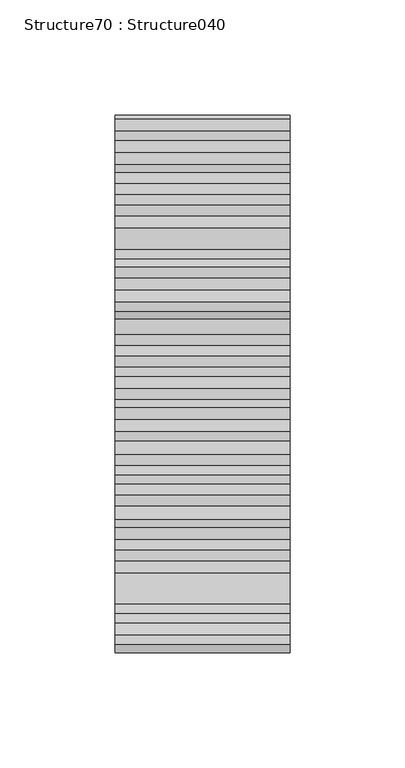
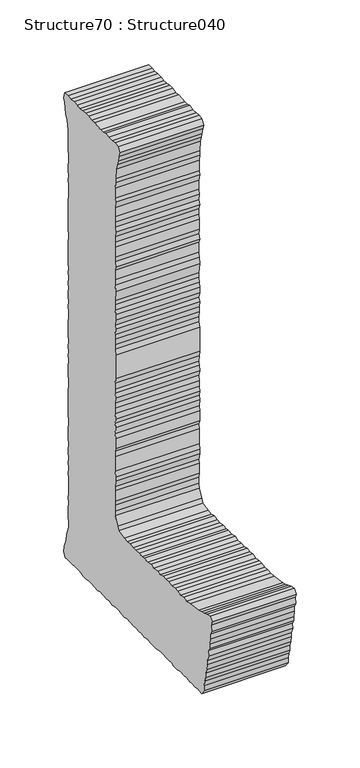
"""IFC4 building model written with IfcOpenShell, lengths in millimetres: proxy geometry, Structure70 : Structure040."""

import ifcopenshell
import ifcopenshell.guid

model = None  # the IFC model being written
_history = None  # IfcOwnerHistory: only IFC2X3 demands one
_inside = {}  # id of a spatial element -> (the spatial element, [elements in it])
_under = {}  # id of a project, library or spatial element -> (it, [spatial elements below it])
_declared = {}  # id of a project -> (the project, [libraries it declares])
_typed = {}  # id of a type object -> (the type object, [elements of that type])
_made_of = {}  # id of a material, layer set ... -> (it, [elements and type objects made of it])


def new_model(schema):
    """Start an empty IFC model of exactly this schema.

    Asked for "IFC4X3", IfcOpenShell would pick the latest addendum, in which some entities
    have other attributes; the version numbers below select the first issue.
    IFC2X3 requires an IfcOwnerHistory on every rooted entity: one is made here for all.
    """
    global model, _history
    if schema == "IFC4X3":
        model = ifcopenshell.file(schema_version=(4, 3, 0, 0))
    else:
        model = ifcopenshell.file(schema=schema)
    _inside.clear()
    _under.clear()
    _declared.clear()
    _typed.clear()
    _made_of.clear()
    _history = None
    if model.schema == "IFC2X3":
        org = make("IfcOrganization", Name="unknown")
        user = make(
            "IfcPersonAndOrganization",
            ThePerson=make("IfcPerson", FamilyName="unknown"),
            TheOrganization=org,
        )
        app = make(
            "IfcApplication",
            ApplicationDeveloper=org,
            Version="unknown",
            ApplicationFullName="unknown",
            ApplicationIdentifier="unknown",
        )
        _history = make(
            "IfcOwnerHistory",
            OwningUser=user,
            OwningApplication=app,
            ChangeAction="ADDED",
            CreationDate=0,
        )
    return model


def make(cls, **values):
    """One entity of the class cls with the attributes given. An attribute that is None is left unset."""
    return model.create_entity(
        cls, **{name: value for name, value in values.items() if value is not None}
    )


def rooted(cls, **values):
    """An entity with a GlobalId (a new one), such as an element, a storey or a relation."""
    return make(cls, GlobalId=ifcopenshell.guid.new(), OwnerHistory=_history, **values)


def si_unit(unit_type, name, prefix=None):
    """IfcSIUnit, for example si_unit("LENGTHUNIT", "METRE", prefix="MILLI")."""
    return make("IfcSIUnit", UnitType=unit_type, Prefix=prefix, Name=name)


def assignment(units):
    """IfcUnitAssignment: the units of a project."""
    return None if units is None else make("IfcUnitAssignment", Units=units)


def point(xyz):
    """IfcCartesianPoint."""
    return None if xyz is None else make("IfcCartesianPoint", Coordinates=xyz)


def direction(xyz):
    """IfcDirection."""
    return None if xyz is None else make("IfcDirection", DirectionRatios=xyz)


def frame(location, z_axis=None, x_axis=None):
    """IfcAxis2Placement3D, a coordinate frame: its origin and axes. An axis left out is left unset."""
    return make(
        "IfcAxis2Placement3D",
        Location=point(location),
        Axis=direction(z_axis),
        RefDirection=direction(x_axis),
    )


def origin():
    """The frame at (0, 0, 0) with its axes left unset."""
    return frame((0.0, 0.0, 0.0))


def place(relative_to, where):
    """IfcLocalPlacement: puts the frame where relative to a parent placement (None: the world)."""
    return make(
        "IfcLocalPlacement", PlacementRelTo=relative_to, RelativePlacement=where
    )


def context(
    kind, dimensions, precision=None, world=None, true_north=None, identifier=None
):
    """IfcGeometricRepresentationContext, for example the 3D "Model" context."""
    return make(
        "IfcGeometricRepresentationContext",
        ContextIdentifier=identifier,
        ContextType=kind,
        CoordinateSpaceDimension=dimensions,
        Precision=precision,
        WorldCoordinateSystem=world,
        TrueNorth=true_north,
    )


def project(units=None, contexts=None):
    """IfcProject with its units and contexts."""
    return rooted(
        "IfcProject",
        Name="project",
        RepresentationContexts=contexts,
        UnitsInContext=assignment(units),
    )


def spatial(cls, under=None, at=None, **own):
    """A site, building, storey or space (cls), placed at a placement, below another one or the project."""
    s = rooted(cls, ObjectPlacement=at, **own)
    if under is not None:
        _under.setdefault(under.id(), (under, []))[1].append(s)
    return s


def polyline(points):
    """IfcPolyline through the points."""
    return make("IfcPolyline", Points=[point(p) for p in points])


def outline(outer, holes=None, kind="AREA"):
    """IfcArbitraryClosedProfileDef: a profile drawn as a closed curve; with holes, ...WithVoids."""
    if holes is None:
        return make("IfcArbitraryClosedProfileDef", ProfileType=kind, OuterCurve=outer)
    return make(
        "IfcArbitraryProfileDefWithVoids",
        ProfileType=kind,
        OuterCurve=outer,
        InnerCurves=holes,
    )


def extrude(swept, where, along, depth):
    """IfcExtrudedAreaSolid: the profile swept, set in the frame where, extruded along a direction by depth."""
    return make(
        "IfcExtrudedAreaSolid",
        SweptArea=swept,
        Position=where,
        ExtrudedDirection=direction(along),
        Depth=depth,
    )


def shape(context_of_items, identifier, shape_type, items):
    """IfcShapeRepresentation: the items that make up one representation, for example the "Body"."""
    return make(
        "IfcShapeRepresentation",
        ContextOfItems=context_of_items,
        RepresentationIdentifier=identifier,
        RepresentationType=shape_type,
        Items=items,
    )


def source(mapping_origin, context_of_items, identifier, shape_type, items):
    """IfcRepresentationMap: a shape defined once, which mapped items show again and again."""
    return make(
        "IfcRepresentationMap",
        MappingOrigin=mapping_origin,
        MappedRepresentation=shape(context_of_items, identifier, shape_type, items),
    )


def transform(
    local_origin,
    x_axis=None,
    y_axis=None,
    z_axis=None,
    scale=None,
    scale2=None,
    scale3=None,
    uniform=True,
):
    """IfcCartesianTransformationOperator3D, or its non-uniform kind. x_axis, y_axis, z_axis: its Axis1, 2, 3."""
    if uniform:
        return make(
            "IfcCartesianTransformationOperator3D",
            Axis1=direction(x_axis),
            Axis2=direction(y_axis),
            LocalOrigin=point(local_origin),
            Scale=scale,
            Axis3=direction(z_axis),
        )
    return make(
        "IfcCartesianTransformationOperator3DnonUniform",
        Axis1=direction(x_axis),
        Axis2=direction(y_axis),
        LocalOrigin=point(local_origin),
        Scale=scale,
        Axis3=direction(z_axis),
        Scale2=scale2,
        Scale3=scale3,
    )


def mapped(mapping_source, mapping_target):
    """IfcMappedItem: shows the shape of a source again, moved by a transform."""
    return make(
        "IfcMappedItem", MappingSource=mapping_source, MappingTarget=mapping_target
    )


def made_of(thing, what):
    """Note that an element or type object is made of a material, layer set ...; save() writes the relation."""
    if what is not None:
        _made_of.setdefault(what.id(), (what, []))[1].append(thing)
    return thing


def element(
    cls,
    number,
    at=None,
    inside=None,
    cuts=None,
    type_object=None,
    material=None,
    context=None,
    identifier="Body",
    shape_type=None,
    held_by="IfcProductDefinitionShape",
    body=None,
    shapes=None,
    **own,
):
    """One element of the class cls, such as IfcWall. Its Tag is "e" and its number.

    at: its placement. inside: the storey or other place that contains it. cuts: it is an
    opening in that element (IfcRelVoidsElement). A single representation is given by context,
    identifier, shape_type and body (its items); several are given by shapes. held_by: the class
    of the entity that holds the representations. save() writes the other relations.
    """
    e = rooted(cls, Tag="e%d" % number, ObjectPlacement=at, **own)
    if body is not None:
        shapes = [shape(context, identifier, shape_type, body)]
    if shapes is not None:
        e.Representation = make(held_by, Representations=shapes)
    if inside is not None:
        _inside.setdefault(inside.id(), (inside, []))[1].append(e)
    if cuts is not None:
        rooted(
            "IfcRelVoidsElement", RelatingBuildingElement=cuts, RelatedOpeningElement=e
        )
    if type_object is not None:
        _typed.setdefault(type_object.id(), (type_object, []))[1].append(e)
    return made_of(e, material)


def aggregate(whole, parts):
    """IfcRelAggregates: a whole, such as a stair, and the parts it consists of."""
    return rooted("IfcRelAggregates", RelatingObject=whole, RelatedObjects=parts)


def save(model, path):
    """Write the relations noted so far, then the file.

    IfcRelAggregates (storeys below a building ...), IfcRelContainedInSpatialStructure (elements
    in a storey), IfcRelDefinesByType, IfcRelAssociatesMaterial and IfcRelDeclares: one each for
    every whole, place, type object, material and project.
    """
    for whole, parts in _under.values():
        aggregate(whole, parts)
    for where, things in _inside.values():
        rooted(
            "IfcRelContainedInSpatialStructure",
            RelatedElements=things,
            RelatingStructure=where,
        )
    for kind, things in _typed.values():
        rooted("IfcRelDefinesByType", RelatedObjects=things, RelatingType=kind)
    for what, things in _made_of.values():
        rooted("IfcRelAssociatesMaterial", RelatedObjects=things, RelatingMaterial=what)
    for by, libraries in _declared.values():
        rooted("IfcRelDeclares", RelatingContext=by, RelatedDefinitions=libraries)
    model.write(path)


def structure70_structure040_d45bf278(model_context):
    return source(origin(), model_context, "Body", "SweptSolid", [
        extrude(outline(polyline([(277613.2824109, 3629.5984101), (277616.8045177, 3633.0980525), (277620.8818178, 3632.5155811), (277626.1866402, 3630.1824862), (277630.2655449, 3628.998288), (277634.3877738, 3627.8397636), (277647.8488009, 3626.0554434), (277653.1311589, 3625.472972), (277657.8326501, 3626.0554434), (277662.5132814, 3625.472972), (277667.7731749, 3626.0554434), (277671.2936772, 3626.6571701), (277677.1552974, 3625.472972), (277681.8343241, 3626.6571701), (277686.5374199, 3626.0554434), (277690.6163245, 3626.6571701), (277694.7385535, 3625.472972), (277699.4191848, 3626.0554434), (277705.280805, 3625.472972), (277709.3805695, 3626.6571701), (277714.640463, 3625.472972), (277719.922821, 3626.0554434), (277723.4433233, 3625.472972), (277728.1239546, 3626.0554434), (277733.3822436, 3625.472972), (277737.5060771, 3625.472972), (277742.1867084, 3626.6571701), (277746.8881996, 3625.472972), (277751.5688309, 3626.0554434), (277760.3492267, 3627.8397636), (277762.1094778, 3631.3410106), (277765.6315847, 3638.9580681), (277766.2108469, 3643.0578326), (277766.2108469, 3648.9258713), (277765.6315847, 3652.9999621), (277765.6315847, 3662.9854159), (277766.2108469, 3666.5027089), (277765.029858, 3672.3691429), (277765.029858, 3676.4432338), (277765.6315847, 3681.7271964), (277765.6315847, 3695.786741), (277766.2108469, 3700.4705815), (277765.029858, 3704.0135482), (277765.029858, 3713.3555556), (277765.6315847, 3718.0554422), (277765.029858, 3723.9154578), (277765.6315847, 3728.0152223), (277765.029858, 3732.1149867), (277765.6315847, 3736.7988273), (277765.6315847, 3742.0747668), (277766.2108469, 3746.7586074), (277765.029858, 3752.04257), (277765.6315847, 3756.7440611), (277766.2108469, 3760.2437036), (277765.6315847, 3766.1021146), (277765.029858, 3770.8036057), (277765.029858, 3793.6451507), (277766.2108469, 3798.3305959), (277766.2108469, 3803.0064134), (277765.6315847, 3808.290376), (277765.6315847, 3812.9726119), (277765.029858, 3818.2309008), (277766.2108469, 3821.7722629), (277765.029858, 3827.0321565), (277765.029858, 3832.3161191), (277765.6315847, 3836.4174882), (277766.2108469, 3841.0900965), (277766.2108469, 3845.1914656), (277765.029858, 3854.5751926), (277765.6315847, 3860.4432313), (277766.2108469, 3865.1190488), (277766.2108469, 3874.5043805), (277765.029858, 3878.0024183), (277766.2108469, 3882.7039095), (277765.6315847, 3887.38775), (277765.6315847, 3896.763454), (277766.2108469, 3901.44569), (277766.2108469, 3906.7328618), (277765.029858, 3911.4054701), (277766.2108469, 3915.5068392), (277765.6315847, 3920.7908018), (277766.2108469, 3925.4746423), (277766.2108469, 3934.2758979), (277765.029858, 3940.1166583), (277765.6315847, 3943.6339514), (277765.6315847, 3953.5937315), (277765.029858, 3958.8776941), (277765.029858, 3962.9774586), (277764.4505958, 3972.3627903), (277762.7112045, 3977.6194746), (277761.5302156, 3981.7208437), (277760.3492267, 3987.0048063), (277758.5889756, 3991.6806238), (277761.5302156, 3995.7803883), (277765.6315847, 3996.9645864), (277770.8898736, 3995.7803883), (277776.1722316, 3995.7803883), (277780.852863, 3996.9645864), (277784.3733652, 3995.7803883), (277788.4747343, 3995.7803883), (277797.8568568, 3996.9645864), (277803.1167503, 3995.7803883), (277807.8182415, 3996.9645864), (277812.4988728, 3996.9645864), (277817.2019686, 3996.390138), (277821.8809953, 3995.7803883), (277825.3806377, 3996.9645864), (277830.6613911, 3996.9645864), (277835.9437491, 3996.390138), (277840.0226537, 3996.9645864), (277845.3034071, 3996.9645864), (277847.0652629, 3991.0788971), (277845.3034071, 3987.5792547), (277844.1448827, 3982.8793681), (277843.5656205, 3977.0209571), (277841.2036426, 3972.9372387), (277840.0226537, 3964.1343784), (277839.465856, 3958.8776941), (277840.0226537, 3953.5937315), (277839.465856, 3950.0940891), (277839.465856, 3945.4182716), (277838.8641293, 3940.718385), (277838.8641293, 3935.4328178), (277839.465856, 3930.1745289), (277839.465856, 3925.4746423), (277838.8641293, 3921.3748778), (277840.0226537, 3916.0909152), (277838.8641293, 3912.5896682), (277838.8641293, 3902.0201384), (277839.465856, 3897.3475301), (277839.465856, 3893.822214), (277840.0226537, 3887.9621984), (277839.465856, 3883.8881076), (277840.0226537, 3879.1769888), (277840.0226537, 3875.0772243), (277839.465856, 3869.2444869), (277838.8641293, 3864.5446004), (277840.0226537, 3855.1769193), (277839.465856, 3850.4754282), (277839.465856, 3846.3772683), (277840.0226537, 3841.6741725), (277839.465856, 3836.4174882), (277838.8641293, 3832.3161191), (277840.0226537, 3827.6162325), (277838.8641293, 3823.5341187), (277839.465856, 3817.6741031), (277838.8641293, 3812.9726119), (277839.465856, 3809.4729695), (277839.465856, 3804.7730829), (277838.8641293, 3800.0876378), (277840.0226537, 3794.8309535), (277838.8641293, 3790.7039107), (277838.8641293, 3784.8438951), (277840.0226537, 3780.7441306), (277839.465856, 3776.0618947), (277840.0226537, 3771.9605256), (277840.0226537, 3767.2590344), (277838.8641293, 3762.5848215), (277839.465856, 3756.7440611), (277838.8641293, 3752.04257), (277840.0226537, 3747.9428055), (277838.8641293, 3743.8414364), (277839.465856, 3737.9750024), (277840.0226537, 3733.2991849), (277840.0226537, 3729.7738688), (277838.8641293, 3724.4979292), (277838.8641293, 3719.2316172), (277839.465856, 3715.1302482), (277839.465856, 3711.0304837), (277840.0226537, 3705.1720727), (277839.465856, 3701.0723082), (277840.0226537, 3696.9709391), (277839.465856, 3691.0868544), (277838.8641293, 3686.4030139), (277838.8641293, 3682.8857208), (277839.465856, 3678.2018803), (277840.0226537, 3672.3691429), (277840.0226537, 3668.8261762), (277838.8641293, 3662.9854159), (277840.0226537, 3658.3015753), (277840.0226537, 3654.7842823), (277838.8641293, 3650.1004418), (277840.0226537, 3644.8245022), (277838.8641293, 3640.7167147), (277839.465856, 3634.856699), (277838.8641293, 3631.3410106), (277838.8641293, 3616.0972679), (277839.465856, 3612.0135494), (277838.8641293, 3607.3393366), (277839.465856, 3602.0280957), (277839.465856, 3598.5284533), (277840.0226537, 3593.2541183), (277838.8641293, 3587.9685511), (277838.8641293, 3583.8864372), (277841.8053693, 3575.0851816), (277842.9638938, 3569.8268927), (277844.1448827, 3565.1254015), (277845.9051338, 3561.025637), (277847.0652629, 3555.7416744), (277844.1448827, 3551.0658569), (277840.6243804, 3551.6675836), (277821.8809953, 3551.6675836), (277816.0193751, 3550.4833855), (277811.3178839, 3550.4833855), (277807.2165148, 3551.6675836), (277803.1167503, 3551.0658569), (277797.8568568, 3551.0658569), (277793.153761, 3550.4833855), (277789.6557232, 3551.6675836), (277784.3733652, 3551.6675836), (277779.0926118, 3551.0658569), (277775.5929694, 3551.6675836), (277770.3330759, 3550.4833855), (277765.029858, 3551.6675836), (277760.3492267, 3551.6675836), (277755.6461309, 3550.4833855), (277751.5688309, 3550.4833855), (277746.8881996, 3551.6675836), (277742.1867084, 3551.0658569), (277736.9268149, 3550.4833855), (277733.3822436, 3551.0658569), (277728.1239546, 3550.4833855), (277724.6243122, 3551.0658569), (277719.922821, 3550.4833855), (277714.640463, 3551.6675836), (277710.539094, 3550.4833855), (277701.1794359, 3550.4833855), (277695.3178157, 3551.6675836), (277690.6163245, 3551.6675836), (277686.5374199, 3551.0658569), (277681.8343241, 3551.0658569), (277677.1552974, 3551.6675836), (277673.6331906, 3550.4833855), (277668.3524372, 3550.4833855), (277663.6718058, 3551.6675836), (277658.3894478, 3551.0658569), (277653.7104211, 3551.6675836), (277649.0297898, 3550.4833855), (277645.5092876, 3551.0658569), (277640.249394, 3550.4833855), (277636.1255605, 3551.6675836), (277630.2655449, 3550.4833855), (277626.1866402, 3555.7416744), (277625.5849135, 3561.025637), (277625.0056513, 3565.7094775), (277623.2454002, 3569.8268927), (277623.2454002, 3574.5107332), (277622.0628067, 3578.6104977), (277620.8818178, 3583.8864372), (277620.8818178, 3587.9685511), (277619.1440311, 3593.2541183), (277619.7457578, 3597.9540049), (277617.38378, 3601.4536473), (277617.38378, 3605.572667), (277616.2027911, 3611.4134274), (277616.2027911, 3616.0972679), (277614.4409353, 3619.6145609), (277615.042662, 3625.472972), (277613.2824109, 3629.5984101)])), frame((-59031.6926606, 0.0, 0.0), z_axis=(1.0, 0.0, 0.0), x_axis=(0.0, 1.0, 0.0)), (0.0, 0.0, 1.0), 76.2),
    ])


if __name__ == "__main__":
    model = new_model("IFC4")
    model_context = context("Model", 3, world=origin())
    ifc_project = project(units=[si_unit("LENGTHUNIT", "METRE", prefix="MILLI")], contexts=[model_context])
    site = spatial("IfcSite", under=ifc_project)
    building = spatial("IfcBuilding", under=site)
    placement = place(None, origin())
    structure70_structure040_shape = structure70_structure040_d45bf278(model_context)
    element("IfcBuildingElementProxy", 1, Name="Structure70 : Structure040", ObjectType="Structure70 : Structure040", at=placement, inside=building, context=model_context, shape_type="MappedRepresentation", body=[
        mapped(structure70_structure040_shape, transform((0.0, 0.0, 0.0), x_axis=(1.0, 0.0, 0.0), y_axis=(0.0, 1.0, 0.0), z_axis=(0.0, 0.0, 1.0))),
    ])
    save(model, "model.ifc")

# Revit data of these elements
# Type "Structure70 : Structure040"
#   NameOverride = "Structure040"
# Element 1 (IfcBuildingElementProxy, "Structure70 : Structure040")
#   Materials on its faces: "BRUSHED ALUM. LETTERING"
# Materials
#   "BRUSHED ALUM. LETTERING": class "Unassigned", colour RGB 169 181 186, transparency 0, Cost = 0
